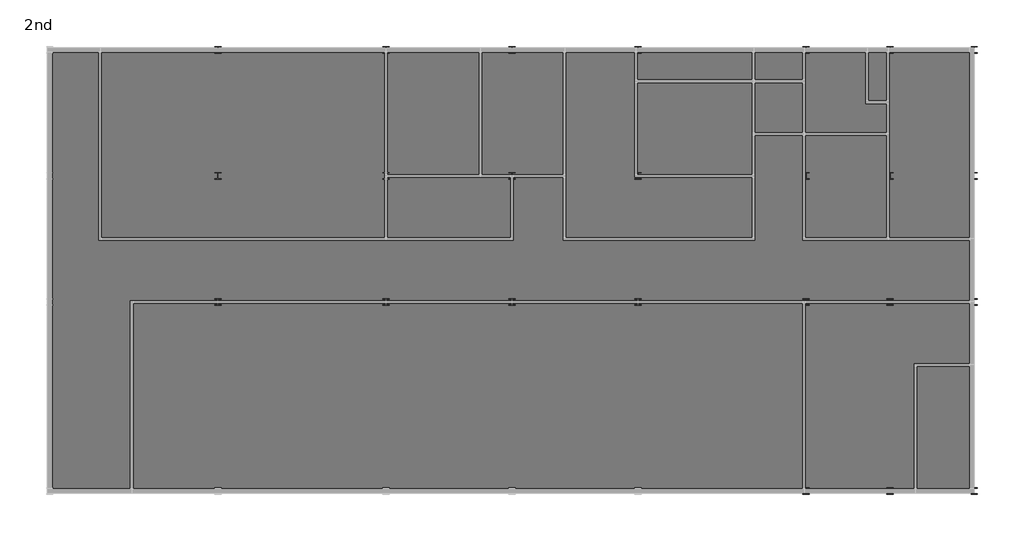
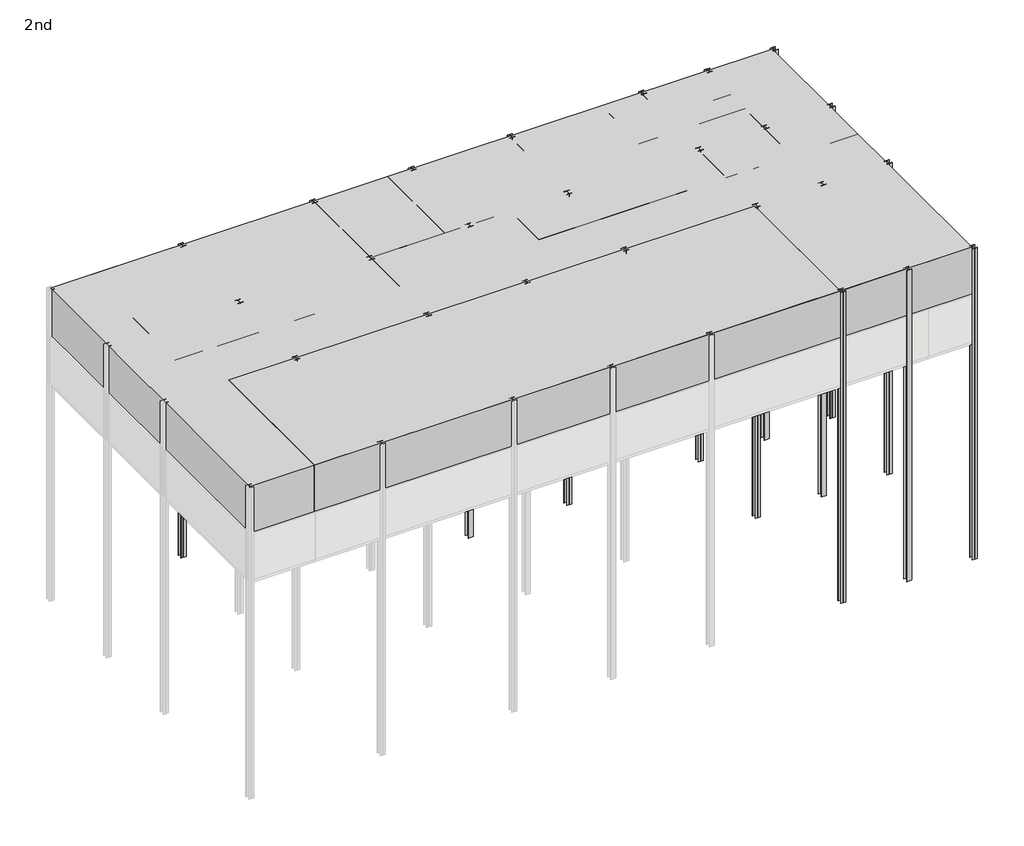
# One storey, part 3 of 3: 18 columns, 17 proxies.
"""IFC4 building model written with IfcOpenShell, lengths in millimetres."""

import ifcopenshell
import ifcopenshell.guid

model = None  # the IFC model being written
_history = None  # IfcOwnerHistory: only IFC2X3 demands one
_inside = {}  # id of a spatial element -> (the spatial element, [elements in it])
_under = {}  # id of a project, library or spatial element -> (it, [spatial elements below it])
_declared = {}  # id of a project -> (the project, [libraries it declares])
_typed = {}  # id of a type object -> (the type object, [elements of that type])
_made_of = {}  # id of a material, layer set ... -> (it, [elements and type objects made of it])


def new_model(schema):
    """Start an empty IFC model of exactly this schema.

    Asked for "IFC4X3", IfcOpenShell would pick the latest addendum, in which some entities
    have other attributes; the version numbers below select the first issue.
    IFC2X3 requires an IfcOwnerHistory on every rooted entity: one is made here for all.
    """
    global model, _history
    if schema == "IFC4X3":
        model = ifcopenshell.file(schema_version=(4, 3, 0, 0))
    else:
        model = ifcopenshell.file(schema=schema)
    _inside.clear()
    _under.clear()
    _declared.clear()
    _typed.clear()
    _made_of.clear()
    _history = None
    if model.schema == "IFC2X3":
        org = make("IfcOrganization", Name="unknown")
        user = make(
            "IfcPersonAndOrganization",
            ThePerson=make("IfcPerson", FamilyName="unknown"),
            TheOrganization=org,
        )
        app = make(
            "IfcApplication",
            ApplicationDeveloper=org,
            Version="unknown",
            ApplicationFullName="unknown",
            ApplicationIdentifier="unknown",
        )
        _history = make(
            "IfcOwnerHistory",
            OwningUser=user,
            OwningApplication=app,
            ChangeAction="ADDED",
            CreationDate=0,
        )
    return model


def make(cls, **values):
    """One entity of the class cls with the attributes given. An attribute that is None is left unset."""
    return model.create_entity(
        cls, **{name: value for name, value in values.items() if value is not None}
    )


def rooted(cls, **values):
    """An entity with a GlobalId (a new one), such as an element, a storey or a relation."""
    return make(cls, GlobalId=ifcopenshell.guid.new(), OwnerHistory=_history, **values)


def si_unit(unit_type, name, prefix=None):
    """IfcSIUnit, for example si_unit("LENGTHUNIT", "METRE", prefix="MILLI")."""
    return make("IfcSIUnit", UnitType=unit_type, Prefix=prefix, Name=name)


def assignment(units):
    """IfcUnitAssignment: the units of a project."""
    return None if units is None else make("IfcUnitAssignment", Units=units)


def point(xyz):
    """IfcCartesianPoint."""
    return None if xyz is None else make("IfcCartesianPoint", Coordinates=xyz)


def direction(xyz):
    """IfcDirection."""
    return None if xyz is None else make("IfcDirection", DirectionRatios=xyz)


def frame(location, z_axis=None, x_axis=None):
    """IfcAxis2Placement3D, a coordinate frame: its origin and axes. An axis left out is left unset."""
    return make(
        "IfcAxis2Placement3D",
        Location=point(location),
        Axis=direction(z_axis),
        RefDirection=direction(x_axis),
    )


def frame_2d(location, x_axis=None):
    """IfcAxis2Placement2D, a coordinate frame in the plane: its origin and x axis."""
    return make(
        "IfcAxis2Placement2D", Location=point(location), RefDirection=direction(x_axis)
    )


def origin():
    """The frame at (0, 0, 0) with its axes left unset."""
    return frame((0.0, 0.0, 0.0))


def origin_with_axes():
    """The frame at (0, 0, 0) with the z axis (0, 0, 1) and the x axis (1, 0, 0) written out."""
    return frame((0.0, 0.0, 0.0), z_axis=(0.0, 0.0, 1.0), x_axis=(1.0, 0.0, 0.0))


def place(relative_to, where):
    """IfcLocalPlacement: puts the frame where relative to a parent placement (None: the world)."""
    return make(
        "IfcLocalPlacement", PlacementRelTo=relative_to, RelativePlacement=where
    )


def context(
    kind, dimensions, precision=None, world=None, true_north=None, identifier=None
):
    """IfcGeometricRepresentationContext, for example the 3D "Model" context."""
    return make(
        "IfcGeometricRepresentationContext",
        ContextIdentifier=identifier,
        ContextType=kind,
        CoordinateSpaceDimension=dimensions,
        Precision=precision,
        WorldCoordinateSystem=world,
        TrueNorth=true_north,
    )


def project(units=None, contexts=None):
    """IfcProject with its units and contexts."""
    return rooted(
        "IfcProject",
        Name="project",
        RepresentationContexts=contexts,
        UnitsInContext=assignment(units),
    )


def spatial(cls, under=None, at=None, **own):
    """A site, building, storey or space (cls), placed at a placement, below another one or the project."""
    s = rooted(cls, ObjectPlacement=at, **own)
    if under is not None:
        _under.setdefault(under.id(), (under, []))[1].append(s)
    return s


def polyline(points):
    """IfcPolyline through the points."""
    return make("IfcPolyline", Points=[point(p) for p in points])


def circle_curve(where, radius):
    """IfcCircle in the frame where."""
    return make("IfcCircle", Position=where, Radius=radius)


def trimmed(basis, trim1, trim2, sense, master):
    """IfcTrimmedCurve: the piece of a basis curve between two trims."""
    return make(
        "IfcTrimmedCurve",
        BasisCurve=basis,
        Trim1=trim1,
        Trim2=trim2,
        SenseAgreement=sense,
        MasterRepresentation=master,
    )


def segment(curve, same_sense, transition):
    """IfcCompositeCurveSegment."""
    return make(
        "IfcCompositeCurveSegment",
        Transition=transition,
        SameSense=same_sense,
        ParentCurve=curve,
    )


def composite_curve(segments, self_intersect=None):
    """IfcCompositeCurve: segments joined end to end."""
    return make("IfcCompositeCurve", Segments=segments, SelfIntersect=self_intersect)


def outline(outer, holes=None, kind="AREA"):
    """IfcArbitraryClosedProfileDef: a profile drawn as a closed curve; with holes, ...WithVoids."""
    if holes is None:
        return make("IfcArbitraryClosedProfileDef", ProfileType=kind, OuterCurve=outer)
    return make(
        "IfcArbitraryProfileDefWithVoids",
        ProfileType=kind,
        OuterCurve=outer,
        InnerCurves=holes,
    )


def extrude(swept, where, along, depth):
    """IfcExtrudedAreaSolid: the profile swept, set in the frame where, extruded along a direction by depth."""
    return make(
        "IfcExtrudedAreaSolid",
        SweptArea=swept,
        Position=where,
        ExtrudedDirection=direction(along),
        Depth=depth,
    )


def shape(context_of_items, identifier, shape_type, items):
    """IfcShapeRepresentation: the items that make up one representation, for example the "Body"."""
    return make(
        "IfcShapeRepresentation",
        ContextOfItems=context_of_items,
        RepresentationIdentifier=identifier,
        RepresentationType=shape_type,
        Items=items,
    )


def source(mapping_origin, context_of_items, identifier, shape_type, items):
    """IfcRepresentationMap: a shape defined once, which mapped items show again and again."""
    return make(
        "IfcRepresentationMap",
        MappingOrigin=mapping_origin,
        MappedRepresentation=shape(context_of_items, identifier, shape_type, items),
    )


def transform(
    local_origin,
    x_axis=None,
    y_axis=None,
    z_axis=None,
    scale=None,
    scale2=None,
    scale3=None,
    uniform=True,
):
    """IfcCartesianTransformationOperator3D, or its non-uniform kind. x_axis, y_axis, z_axis: its Axis1, 2, 3."""
    if uniform:
        return make(
            "IfcCartesianTransformationOperator3D",
            Axis1=direction(x_axis),
            Axis2=direction(y_axis),
            LocalOrigin=point(local_origin),
            Scale=scale,
            Axis3=direction(z_axis),
        )
    return make(
        "IfcCartesianTransformationOperator3DnonUniform",
        Axis1=direction(x_axis),
        Axis2=direction(y_axis),
        LocalOrigin=point(local_origin),
        Scale=scale,
        Axis3=direction(z_axis),
        Scale2=scale2,
        Scale3=scale3,
    )


def mapped(mapping_source, mapping_target):
    """IfcMappedItem: shows the shape of a source again, moved by a transform."""
    return make(
        "IfcMappedItem", MappingSource=mapping_source, MappingTarget=mapping_target
    )


def made_of(thing, what):
    """Note that an element or type object is made of a material, layer set ...; save() writes the relation."""
    if what is not None:
        _made_of.setdefault(what.id(), (what, []))[1].append(thing)
    return thing


def element(
    cls,
    number,
    at=None,
    inside=None,
    cuts=None,
    type_object=None,
    material=None,
    context=None,
    identifier="Body",
    shape_type=None,
    held_by="IfcProductDefinitionShape",
    body=None,
    shapes=None,
    **own,
):
    """One element of the class cls, such as IfcWall. Its Tag is "e" and its number.

    at: its placement. inside: the storey or other place that contains it. cuts: it is an
    opening in that element (IfcRelVoidsElement). A single representation is given by context,
    identifier, shape_type and body (its items); several are given by shapes. held_by: the class
    of the entity that holds the representations. save() writes the other relations.
    """
    e = rooted(cls, Tag="e%d" % number, ObjectPlacement=at, **own)
    if body is not None:
        shapes = [shape(context, identifier, shape_type, body)]
    if shapes is not None:
        e.Representation = make(held_by, Representations=shapes)
    if inside is not None:
        _inside.setdefault(inside.id(), (inside, []))[1].append(e)
    if cuts is not None:
        rooted(
            "IfcRelVoidsElement", RelatingBuildingElement=cuts, RelatedOpeningElement=e
        )
    if type_object is not None:
        _typed.setdefault(type_object.id(), (type_object, []))[1].append(e)
    return made_of(e, material)


def aggregate(whole, parts):
    """IfcRelAggregates: a whole, such as a stair, and the parts it consists of."""
    return rooted("IfcRelAggregates", RelatingObject=whole, RelatedObjects=parts)


def save(model, path):
    """Write the relations noted so far, then the file.

    IfcRelAggregates (storeys below a building ...), IfcRelContainedInSpatialStructure (elements
    in a storey), IfcRelDefinesByType, IfcRelAssociatesMaterial and IfcRelDeclares: one each for
    every whole, place, type object, material and project.
    """
    for whole, parts in _under.values():
        aggregate(whole, parts)
    for where, things in _inside.values():
        rooted(
            "IfcRelContainedInSpatialStructure",
            RelatedElements=things,
            RelatingStructure=where,
        )
    for kind, things in _typed.values():
        rooted("IfcRelDefinesByType", RelatedObjects=things, RelatingType=kind)
    for what, things in _made_of.values():
        rooted("IfcRelAssociatesMaterial", RelatedObjects=things, RelatingMaterial=what)
    for by, libraries in _declared.values():
        rooted("IfcRelDeclares", RelatingContext=by, RelatedDefinitions=libraries)
    model.write(path)


def generic_models_29bcd6f9(model_context):
    return source(origin(), model_context, "Body", "SweptSolid", [
        extrude(outline(polyline([(2000.0, 4500.0), (2000.0, -4500.0), (-2000.0, -4500.0), (-2000.0, 4500.0), (2000.0, 4500.0)])), origin_with_axes(), (0.0, 0.0, 1.0), 6000.0),
    ])


def generic_models_5634f436(model_context):
    return source(origin(), model_context, "Body", "SweptSolid", [
        extrude(outline(polyline([(1350.0, 3000.0), (1350.0, -3000.0), (-1350.0, -3000.0), (-1350.0, 3000.0), (1350.0, 3000.0)])), origin_with_axes(), (0.0, 0.0, 1.0), 6000.0),
    ])


def generic_models_71e2440f(model_context):
    return source(origin(), model_context, "Body", "SweptSolid", [
        extrude(outline(polyline([(500.0, 1250.0), (500.0, -1250.0), (-500.0, -1250.0), (-500.0, 1250.0), (500.0, 1250.0)])), origin_with_axes(), (0.0, 0.0, 1.0), 6000.0),
    ])


def generic_models_57c7875f(model_context):
    return source(origin(), model_context, "Body", "SweptSolid", [
        extrude(outline(polyline([(4500.0, 16000.0), (4500.0, -16000.0), (-4500.0, -16000.0), (-4500.0, 16000.0), (4500.0, 16000.0)])), origin_with_axes(), (0.0, 0.0, 1.0), 6000.0),
    ])


def generic_models_7bff30ad(model_context):
    return source(origin(), model_context, "Body", "SweptSolid", [
        extrude(outline(polyline([(2000.0, 2000.0), (2000.0, -2000.0), (-2000.0, -2000.0), (-2000.0, 2000.0), (2000.0, 2000.0)])), origin_with_axes(), (0.0, 0.0, 1.0), 6000.0),
    ])


def generic_models_5b7b272c(model_context):
    return source(origin(), model_context, "Body", "SweptSolid", [
        extrude(outline(polyline([(2000.0, 2500.0), (2000.0, -2500.0), (-2000.0, -2500.0), (-2000.0, 2500.0), (2000.0, 2500.0)])), origin_with_axes(), (0.0, 0.0, 1.0), 6000.0),
    ])


def generic_models_47b98be1(model_context):
    return source(origin(), model_context, "Body", "SweptSolid", [
        extrude(outline(polyline([(1200.0, 2000.0), (1200.0, -2000.0), (-1200.0, -2000.0), (-1200.0, 2000.0), (1200.0, 2000.0)])), origin_with_axes(), (0.0, 0.0, 1.0), 6000.0),
    ])


def generic_models_7a053eeb(model_context):
    return source(origin(), model_context, "Body", "SweptSolid", [
        extrude(outline(polyline([(1200.0, 750.0), (1200.0, -750.0), (-1200.0, -750.0), (-1200.0, 750.0), (1200.0, 750.0)])), origin_with_axes(), (0.0, 0.0, 1.0), 6000.0),
    ])


def generic_models_ec17d728(model_context):
    return source(origin(), model_context, "Body", "SweptSolid", [
        extrude(outline(polyline([(2800.0, 3000.0), (2800.0, -3000.0), (-2800.0, -3000.0), (-2800.0, 3000.0), (2800.0, 3000.0)])), origin_with_axes(), (0.0, 0.0, 1.0), 6000.0),
    ])


def generic_models_85897e09(model_context):
    return source(origin(), model_context, "Body", "SweptSolid", [
        extrude(outline(polyline([(2800.0, 750.0), (2800.0, -750.0), (-2800.0, -750.0), (-2800.0, 750.0), (2800.0, 750.0)])), origin_with_axes(), (0.0, 0.0, 1.0), 6000.0),
    ])


def generic_models_b79df083(model_context):
    return source(origin(), model_context, "Body", "SweptSolid", [
        extrude(outline(polyline([(4500.0, 4500.0), (4500.0, -4500.0), (-4500.0, -4500.0), (-4500.0, 4500.0), (4500.0, 4500.0)])), origin_with_axes(), (0.0, 0.0, 1.0), 6000.0),
    ])


def generic_models_98b71764(model_context):
    return source(origin(), model_context, "Body", "SweptSolid", [
        extrude(outline(polyline([(2000.0, 3000.0), (2000.0, -3000.0), (-2000.0, -3000.0), (-2000.0, 3000.0), (2000.0, 3000.0)])), origin_with_axes(), (0.0, 0.0, 1.0), 6000.0),
    ])


def generic_models_8af91fed(model_context):
    return source(origin(), model_context, "Body", "SweptSolid", [
        extrude(outline(polyline([(2250.0, 3000.0), (2250.0, -3000.0), (-2250.0, -3000.0), (-2250.0, 3000.0), (2250.0, 3000.0)])), origin_with_axes(), (0.0, 0.0, 1.0), 6000.0),
    ])


def generic_models_542cc789(model_context):
    return source(origin(), model_context, "Body", "SweptSolid", [
        extrude(outline(polyline([(1500.0, 3000.0), (1500.0, -3000.0), (-1500.0, -3000.0), (-1500.0, 3000.0), (1500.0, 3000.0)])), origin_with_axes(), (0.0, 0.0, 1.0), 6000.0),
    ])


def generic_models_af0009da(model_context):
    return source(origin(), model_context, "Body", "SweptSolid", [
        extrude(outline(polyline([(4500.0, 6800.0), (4500.0, -6800.0), (-4500.0, -6800.0), (-4500.0, 6800.0), (4500.0, 6800.0)])), origin_with_axes(), (0.0, 0.0, 1.0), 6000.0),
    ])


def generic_models_4d084078(model_context):
    return source(origin(), model_context, "Body", "SweptSolid", [
        extrude(outline(polyline([(4000.0, 4500.0), (4000.0, -4500.0), (-4000.0, -4500.0), (-4000.0, 4500.0), (4000.0, 4500.0)])), origin_with_axes(), (0.0, 0.0, 1.0), 6000.0),
    ])


def generic_models_b3b0fa1d(model_context):
    return source(origin(), model_context, "Body", "SweptSolid", [
        extrude(outline(polyline([(21950.0, 10500.0), (21950.0, -10500.0), (-21950.0, -10500.0), (-21950.0, 10500.0), (21950.0, 10500.0)])), origin_with_axes(), (0.0, 0.0, 1.0), 6000.0),
    ])


model = new_model("IFC4")

# Units and contexts
model_context = context("Model", 3, world=origin())
ifc_project = project(units=[si_unit("LENGTHUNIT", "METRE", prefix="MILLI")], contexts=[model_context])

# Site, building, storey
site = spatial("IfcSite", under=ifc_project)
building = spatial("IfcBuilding", under=site)
storey = spatial("IfcBuildingStorey", under=building, Name="2nd", Elevation=14000.0)

# Proxies
placement = place(None, origin())
generic_models_shape = generic_models_29bcd6f9(model_context)
element("IfcBuildingElementProxy", 1, Name="Space Planning Box_hec : Space Planning Box_hec", ObjectType="Space Planning Box_hec : Space Planning Box_hec", at=placement, inside=storey, context=model_context, shape_type="MappedRepresentation", body=[
    mapped(generic_models_shape, transform((198014.1020501, 147515.7581198, 14000.0), x_axis=(1.0, 0.0, 0.0), y_axis=(0.0, 1.0, 0.0), z_axis=(0.0, 0.0, 1.0))),
])
generic_models_2_shape = generic_models_5634f436(model_context)
element("IfcBuildingElementProxy", 2, Name="Space Planning Box_hec : Space Planning Box_hec", ObjectType="Space Planning Box_hec : Space Planning Box_hec", at=placement, inside=storey, context=model_context, shape_type="MappedRepresentation", body=[
    mapped(generic_models_2_shape, transform((198664.1020501, 134015.7581198, 14000.0), x_axis=(1.0, 0.0, 0.0), y_axis=(0.0, 1.0, 0.0), z_axis=(0.0, 0.0, 1.0))),
])
generic_models_3_shape = generic_models_71e2440f(model_context)
element("IfcBuildingElementProxy", 3, Name="Space Planning Box_hec : Space Planning Box_hec", ObjectType="Space Planning Box_hec : Space Planning Box_hec", at=placement, inside=storey, context=model_context, shape_type="MappedRepresentation", body=[
    mapped(generic_models_3_shape, transform((195514.1020501, 150765.7581198, 14000.0), x_axis=(1.0, 0.0, 0.0), y_axis=(0.0, 1.0, 0.0), z_axis=(0.0, 0.0, 1.0))),
])
generic_models_4_shape = generic_models_57c7875f(model_context)
element("IfcBuildingElementProxy", 4, Name="Space Planning Box_hec : Space Planning Box_hec", ObjectType="Space Planning Box_hec : Space Planning Box_hec", at=placement, inside=storey, context=model_context, shape_type="MappedRepresentation", body=[
    mapped(generic_models_4_shape, transform((176014.1020501, 135515.7581198, 14000.0), x_axis=(0.0, -1.0, 0.0), y_axis=(1.0, 0.0, 0.0), z_axis=(0.0, 0.0, 1.0))),
])
generic_models_5_shape = generic_models_7bff30ad(model_context)
element("IfcBuildingElementProxy", 5, Name="Space Planning Box_hec : Space Planning Box_hec", ObjectType="Space Planning Box_hec : Space Planning Box_hec", at=placement, inside=storey, context=model_context, shape_type="MappedRepresentation", body=[
    mapped(generic_models_5_shape, transform((194014.1020501, 150015.7581198, 14000.0), x_axis=(1.0, 0.0, 0.0), y_axis=(0.0, 1.0, 0.0), z_axis=(0.0, 0.0, 1.0))),
])
generic_models_6_shape = generic_models_5b7b272c(model_context)
element("IfcBuildingElementProxy", 6, Name="Space Planning Box_hec : Space Planning Box_hec", ObjectType="Space Planning Box_hec : Space Planning Box_hec", at=placement, inside=storey, context=model_context, shape_type="MappedRepresentation", body=[
    mapped(generic_models_6_shape, transform((194014.1020501, 145515.7581198, 14000.0), x_axis=(1.0, 0.0, 0.0), y_axis=(0.0, 1.0, 0.0), z_axis=(0.0, 0.0, 1.0))),
])
generic_models_7_shape = generic_models_47b98be1(model_context)
element("IfcBuildingElementProxy", 7, Name="Space Planning Box_hec : Space Planning Box_hec", ObjectType="Space Planning Box_hec : Space Planning Box_hec", at=placement, inside=storey, context=model_context, shape_type="MappedRepresentation", body=[
    mapped(generic_models_7_shape, transform((190814.1020501, 150015.7581198, 14000.0), x_axis=(1.0, 0.0, 0.0), y_axis=(0.0, 1.0, 0.0), z_axis=(0.0, 0.0, 1.0))),
])
generic_models_8_shape = generic_models_7a053eeb(model_context)
element("IfcBuildingElementProxy", 8, Name="Space Planning Box_hec : Space Planning Box_hec", ObjectType="Space Planning Box_hec : Space Planning Box_hec", at=placement, inside=storey, context=model_context, shape_type="MappedRepresentation", body=[
    mapped(generic_models_8_shape, transform((190814.1020501, 151265.7581198, 14000.0), x_axis=(1.0, 0.0, 0.0), y_axis=(0.0, 1.0, 0.0), z_axis=(0.0, 0.0, 1.0))),
])
generic_models_9_shape = generic_models_ec17d728(model_context)
element("IfcBuildingElementProxy", 9, Name="Space Planning Box_hec : Space Planning Box_hec", ObjectType="Space Planning Box_hec : Space Planning Box_hec", at=placement, inside=storey, context=model_context, shape_type="MappedRepresentation", body=[
    mapped(generic_models_9_shape, transform((186814.1020501, 149015.7581198, 14000.0), x_axis=(1.0, 0.0, 0.0), y_axis=(0.0, 1.0, 0.0), z_axis=(0.0, 0.0, 1.0))),
])
generic_models_10_shape = generic_models_85897e09(model_context)
element("IfcBuildingElementProxy", 10, Name="Space Planning Box_hec : Space Planning Box_hec", ObjectType="Space Planning Box_hec : Space Planning Box_hec", at=placement, inside=storey, context=model_context, shape_type="MappedRepresentation", body=[
    mapped(generic_models_10_shape, transform((186814.1020501, 151265.7581198, 14000.0), x_axis=(1.0, 0.0, 0.0), y_axis=(0.0, 1.0, 0.0), z_axis=(0.0, 0.0, 1.0))),
])
generic_models_11_shape = generic_models_b79df083(model_context)
element("IfcBuildingElementProxy", 11, Name="Space Planning Box_hec : Space Planning Box_hec", ObjectType="Space Planning Box_hec : Space Planning Box_hec", at=placement, inside=storey, context=model_context, shape_type="MappedRepresentation", body=[
    mapped(generic_models_11_shape, transform((185114.1020501, 147515.7581198, 14000.0), x_axis=(1.0, 0.0, 0.0), y_axis=(0.0, 1.0, 0.0), z_axis=(0.0, 0.0, 1.0))),
])
generic_models_12_shape = generic_models_98b71764(model_context)
element("IfcBuildingElementProxy", 12, Name="Space Planning Box_hec : Space Planning Box_hec", ObjectType="Space Planning Box_hec : Space Planning Box_hec", at=placement, inside=storey, context=model_context, shape_type="MappedRepresentation", body=[
    mapped(generic_models_12_shape, transform((178614.1020501, 149015.7581198, 14000.0), x_axis=(1.0, 0.0, 0.0), y_axis=(0.0, 1.0, 0.0), z_axis=(0.0, 0.0, 1.0))),
])
generic_models_13_shape = generic_models_8af91fed(model_context)
element("IfcBuildingElementProxy", 13, Name="Space Planning Box_hec : Space Planning Box_hec", ObjectType="Space Planning Box_hec : Space Planning Box_hec", at=placement, inside=storey, context=model_context, shape_type="MappedRepresentation", body=[
    mapped(generic_models_13_shape, transform((174364.1020501, 149015.7581198, 14000.0), x_axis=(1.0, 0.0, 0.0), y_axis=(0.0, 1.0, 0.0), z_axis=(0.0, 0.0, 1.0))),
])
generic_models_14_shape = generic_models_542cc789(model_context)
element("IfcBuildingElementProxy", 14, Name="Space Planning Box_hec : Space Planning Box_hec", ObjectType="Space Planning Box_hec : Space Planning Box_hec", at=placement, inside=storey, context=model_context, shape_type="MappedRepresentation", body=[
    mapped(generic_models_14_shape, transform((175114.1020501, 144515.7581198, 14000.0), x_axis=(0.0, 1.0, 0.0), y_axis=(-1.0, 0.0, 0.0), z_axis=(0.0, 0.0, 1.0))),
])
generic_models_15_shape = generic_models_af0009da(model_context)
element("IfcBuildingElementProxy", 15, Name="Space Planning Box_hec : Space Planning Box_hec", ObjectType="Space Planning Box_hec : Space Planning Box_hec", at=placement, inside=storey, context=model_context, shape_type="MappedRepresentation", body=[
    mapped(generic_models_15_shape, transform((165314.1020501, 147515.7581198, 14000.0), x_axis=(0.0, -1.0, 0.0), y_axis=(1.0, 0.0, 0.0), z_axis=(0.0, 0.0, 1.0))),
])
generic_models_16_shape = generic_models_4d084078(model_context)
element("IfcBuildingElementProxy", 16, Name="Space Planning Box_hec : Space Planning Box_hec", ObjectType="Space Planning Box_hec : Space Planning Box_hec", at=placement, inside=storey, context=model_context, shape_type="MappedRepresentation", body=[
    mapped(generic_models_16_shape, transform((196014.1020501, 135515.7581198, 14000.0), x_axis=(1.0, 0.0, 0.0), y_axis=(0.0, 1.0, 0.0), z_axis=(0.0, 0.0, 1.0))),
])
generic_models_17_shape = generic_models_b3b0fa1d(model_context)
element("IfcBuildingElementProxy", 17, Name="Space Planning Box_hec : Space Planning Box_hec", ObjectType="Space Planning Box_hec : Space Planning Box_hec", at=placement, inside=storey, context=model_context, shape_type="MappedRepresentation", body=[
    mapped(generic_models_17_shape, transform((178064.1020501, 141515.7581198, 14000.0), x_axis=(1.0, 0.0, 0.0), y_axis=(0.0, 1.0, 0.0), z_axis=(0.0, 0.0, 1.0))),
])

# Columns
element("IfcColumn", 18, ObjectType="UC-Universal Columns-Column : UC305x305x97", at=placement, inside=storey, context=model_context, shape_type="SweptSolid", body=[
    extrude(outline(composite_curve([segment(polyline([(164266.7520501, 152169.7081198), (164266.7520501, 152154.3081198), (164134.2520501, 152154.3081198)]), True, "CONTINUOUS"), segment(trimmed(circle_curve(frame_2d((164134.2520501, 152139.1081198)), 15.2), [point((164134.2520501, 152154.3081198))], [point((164119.0520501, 152139.1081198))], True, "CARTESIAN"), True, "CONTINUOUS"), segment(polyline([(164119.0520501, 152139.1081198), (164119.0520501, 151892.4081198)]), True, "CONTINUOUS"), segment(trimmed(circle_curve(frame_2d((164134.2520501, 151892.4081198)), 15.2), [point((164119.0520501, 151892.4081198))], [point((164134.2520501, 151877.2081198))], True, "CARTESIAN"), True, "CONTINUOUS"), segment(polyline([(164134.2520501, 151877.2081198), (164266.7520501, 151877.2081198), (164266.7520501, 151861.8081198), (163961.4520501, 151861.8081198), (163961.4520501, 151877.2081198), (164093.9520501, 151877.2081198)]), True, "CONTINUOUS"), segment(trimmed(circle_curve(frame_2d((164093.9520501, 151892.4081198)), 15.2), [point((164093.9520501, 151877.2081198))], [point((164109.1520501, 151892.4081198))], True, "CARTESIAN"), True, "CONTINUOUS"), segment(polyline([(164109.1520501, 151892.4081198), (164109.1520501, 152139.1081198)]), True, "CONTINUOUS"), segment(trimmed(circle_curve(frame_2d((164093.9520501, 152139.1081198)), 15.2), [point((164109.1520501, 152139.1081198))], [point((164093.9520501, 152154.3081198))], True, "CARTESIAN"), True, "CONTINUOUS"), segment(polyline([(164093.9520501, 152154.3081198), (163961.4520501, 152154.3081198), (163961.4520501, 152169.7081198), (164266.7520501, 152169.7081198)]), True, "CONTINUOUS")], self_intersect=False)), origin_with_axes(), (0.0, 0.0, 1.0), 20000.0),
])
element("IfcColumn", 19, ObjectType="UC-Universal Columns-Column : UC305x305x97", at=placement, inside=storey, context=model_context, shape_type="SweptSolid", body=[
    extrude(outline(composite_curve([segment(polyline([(172266.7520501, 152169.7081198), (172266.7520501, 152154.3081198), (172134.2520501, 152154.3081198)]), True, "CONTINUOUS"), segment(trimmed(circle_curve(frame_2d((172134.2520501, 152139.1081198)), 15.2), [point((172134.2520501, 152154.3081198))], [point((172119.0520501, 152139.1081198))], True, "CARTESIAN"), True, "CONTINUOUS"), segment(polyline([(172119.0520501, 152139.1081198), (172119.0520501, 151892.4081198)]), True, "CONTINUOUS"), segment(trimmed(circle_curve(frame_2d((172134.2520501, 151892.4081198)), 15.2), [point((172119.0520501, 151892.4081198))], [point((172134.2520501, 151877.2081198))], True, "CARTESIAN"), True, "CONTINUOUS"), segment(polyline([(172134.2520501, 151877.2081198), (172266.7520501, 151877.2081198), (172266.7520501, 151861.8081198), (171961.4520501, 151861.8081198), (171961.4520501, 151877.2081198), (172093.9520501, 151877.2081198)]), True, "CONTINUOUS"), segment(trimmed(circle_curve(frame_2d((172093.9520501, 151892.4081198)), 15.2), [point((172093.9520501, 151877.2081198))], [point((172109.1520501, 151892.4081198))], True, "CARTESIAN"), True, "CONTINUOUS"), segment(polyline([(172109.1520501, 151892.4081198), (172109.1520501, 152139.1081198)]), True, "CONTINUOUS"), segment(trimmed(circle_curve(frame_2d((172093.9520501, 152139.1081198)), 15.2), [point((172109.1520501, 152139.1081198))], [point((172093.9520501, 152154.3081198))], True, "CARTESIAN"), True, "CONTINUOUS"), segment(polyline([(172093.9520501, 152154.3081198), (171961.4520501, 152154.3081198), (171961.4520501, 152169.7081198), (172266.7520501, 152169.7081198)]), True, "CONTINUOUS")], self_intersect=False)), origin_with_axes(), (0.0, 0.0, 1.0), 20000.0),
])
element("IfcColumn", 20, ObjectType="UC-Universal Columns-Column : UC305x305x97", at=placement, inside=storey, context=model_context, shape_type="SweptSolid", body=[
    extrude(outline(composite_curve([segment(polyline([(178266.7520501, 152169.7081198), (178266.7520501, 152154.3081198), (178134.2520501, 152154.3081198)]), True, "CONTINUOUS"), segment(trimmed(circle_curve(frame_2d((178134.2520501, 152139.1081198)), 15.2), [point((178134.2520501, 152154.3081198))], [point((178119.0520501, 152139.1081198))], True, "CARTESIAN"), True, "CONTINUOUS"), segment(polyline([(178119.0520501, 152139.1081198), (178119.0520501, 151892.4081198)]), True, "CONTINUOUS"), segment(trimmed(circle_curve(frame_2d((178134.2520501, 151892.4081198)), 15.2), [point((178119.0520501, 151892.4081198))], [point((178134.2520501, 151877.2081198))], True, "CARTESIAN"), True, "CONTINUOUS"), segment(polyline([(178134.2520501, 151877.2081198), (178266.7520501, 151877.2081198), (178266.7520501, 151861.8081198), (177961.4520501, 151861.8081198), (177961.4520501, 151877.2081198), (178093.9520501, 151877.2081198)]), True, "CONTINUOUS"), segment(trimmed(circle_curve(frame_2d((178093.9520501, 151892.4081198)), 15.2), [point((178093.9520501, 151877.2081198))], [point((178109.1520501, 151892.4081198))], True, "CARTESIAN"), True, "CONTINUOUS"), segment(polyline([(178109.1520501, 151892.4081198), (178109.1520501, 152139.1081198)]), True, "CONTINUOUS"), segment(trimmed(circle_curve(frame_2d((178093.9520501, 152139.1081198)), 15.2), [point((178109.1520501, 152139.1081198))], [point((178093.9520501, 152154.3081198))], True, "CARTESIAN"), True, "CONTINUOUS"), segment(polyline([(178093.9520501, 152154.3081198), (177961.4520501, 152154.3081198), (177961.4520501, 152169.7081198), (178266.7520501, 152169.7081198)]), True, "CONTINUOUS")], self_intersect=False)), origin_with_axes(), (0.0, 0.0, 1.0), 20000.0),
])
element("IfcColumn", 21, ObjectType="UC-Universal Columns-Column : UC305x305x97", at=placement, inside=storey, context=model_context, shape_type="SweptSolid", body=[
    extrude(outline(composite_curve([segment(polyline([(178266.7520501, 146169.7081198), (178266.7520501, 146154.3081198), (178134.2520501, 146154.3081198)]), True, "CONTINUOUS"), segment(trimmed(circle_curve(frame_2d((178134.2520501, 146139.1081198)), 15.2), [point((178134.2520501, 146154.3081198))], [point((178119.0520501, 146139.1081198))], True, "CARTESIAN"), True, "CONTINUOUS"), segment(polyline([(178119.0520501, 146139.1081198), (178119.0520501, 145892.4081198)]), True, "CONTINUOUS"), segment(trimmed(circle_curve(frame_2d((178134.2520501, 145892.4081198)), 15.2), [point((178119.0520501, 145892.4081198))], [point((178134.2520501, 145877.2081198))], True, "CARTESIAN"), True, "CONTINUOUS"), segment(polyline([(178134.2520501, 145877.2081198), (178266.7520501, 145877.2081198), (178266.7520501, 145861.8081198), (177961.4520501, 145861.8081198), (177961.4520501, 145877.2081198), (178093.9520501, 145877.2081198)]), True, "CONTINUOUS"), segment(trimmed(circle_curve(frame_2d((178093.9520501, 145892.4081198)), 15.2), [point((178093.9520501, 145877.2081198))], [point((178109.1520501, 145892.4081198))], True, "CARTESIAN"), True, "CONTINUOUS"), segment(polyline([(178109.1520501, 145892.4081198), (178109.1520501, 146139.1081198)]), True, "CONTINUOUS"), segment(trimmed(circle_curve(frame_2d((178093.9520501, 146139.1081198)), 15.2), [point((178109.1520501, 146139.1081198))], [point((178093.9520501, 146154.3081198))], True, "CARTESIAN"), True, "CONTINUOUS"), segment(polyline([(178093.9520501, 146154.3081198), (177961.4520501, 146154.3081198), (177961.4520501, 146169.7081198), (178266.7520501, 146169.7081198)]), True, "CONTINUOUS")], self_intersect=False)), origin_with_axes(), (0.0, 0.0, 1.0), 20000.0),
])
element("IfcColumn", 22, ObjectType="UC-Universal Columns-Column : UC305x305x97", at=placement, inside=storey, context=model_context, shape_type="SweptSolid", body=[
    extrude(outline(composite_curve([segment(polyline([(184266.7520501, 152169.7081198), (184266.7520501, 152154.3081198), (184134.2520501, 152154.3081198)]), True, "CONTINUOUS"), segment(trimmed(circle_curve(frame_2d((184134.2520501, 152139.1081198)), 15.2), [point((184134.2520501, 152154.3081198))], [point((184119.0520501, 152139.1081198))], True, "CARTESIAN"), True, "CONTINUOUS"), segment(polyline([(184119.0520501, 152139.1081198), (184119.0520501, 151892.4081198)]), True, "CONTINUOUS"), segment(trimmed(circle_curve(frame_2d((184134.2520501, 151892.4081198)), 15.2), [point((184119.0520501, 151892.4081198))], [point((184134.2520501, 151877.2081198))], True, "CARTESIAN"), True, "CONTINUOUS"), segment(polyline([(184134.2520501, 151877.2081198), (184266.7520501, 151877.2081198), (184266.7520501, 151861.8081198), (183961.4520501, 151861.8081198), (183961.4520501, 151877.2081198), (184093.9520501, 151877.2081198)]), True, "CONTINUOUS"), segment(trimmed(circle_curve(frame_2d((184093.9520501, 151892.4081198)), 15.2), [point((184093.9520501, 151877.2081198))], [point((184109.1520501, 151892.4081198))], True, "CARTESIAN"), True, "CONTINUOUS"), segment(polyline([(184109.1520501, 151892.4081198), (184109.1520501, 152139.1081198)]), True, "CONTINUOUS"), segment(trimmed(circle_curve(frame_2d((184093.9520501, 152139.1081198)), 15.2), [point((184109.1520501, 152139.1081198))], [point((184093.9520501, 152154.3081198))], True, "CARTESIAN"), True, "CONTINUOUS"), segment(polyline([(184093.9520501, 152154.3081198), (183961.4520501, 152154.3081198), (183961.4520501, 152169.7081198), (184266.7520501, 152169.7081198)]), True, "CONTINUOUS")], self_intersect=False)), origin_with_axes(), (0.0, 0.0, 1.0), 20000.0),
])
element("IfcColumn", 23, ObjectType="UC-Universal Columns-Column : UC305x305x97", at=placement, inside=storey, context=model_context, shape_type="SweptSolid", body=[
    extrude(outline(composite_curve([segment(polyline([(184266.7520501, 146169.7081198), (184266.7520501, 146154.3081198), (184134.2520501, 146154.3081198)]), True, "CONTINUOUS"), segment(trimmed(circle_curve(frame_2d((184134.2520501, 146139.1081198)), 15.2), [point((184134.2520501, 146154.3081198))], [point((184119.0520501, 146139.1081198))], True, "CARTESIAN"), True, "CONTINUOUS"), segment(polyline([(184119.0520501, 146139.1081198), (184119.0520501, 145892.4081198)]), True, "CONTINUOUS"), segment(trimmed(circle_curve(frame_2d((184134.2520501, 145892.4081198)), 15.2), [point((184119.0520501, 145892.4081198))], [point((184134.2520501, 145877.2081198))], True, "CARTESIAN"), True, "CONTINUOUS"), segment(polyline([(184134.2520501, 145877.2081198), (184266.7520501, 145877.2081198), (184266.7520501, 145861.8081198), (183961.4520501, 145861.8081198), (183961.4520501, 145877.2081198), (184093.9520501, 145877.2081198)]), True, "CONTINUOUS"), segment(trimmed(circle_curve(frame_2d((184093.9520501, 145892.4081198)), 15.2), [point((184093.9520501, 145877.2081198))], [point((184109.1520501, 145892.4081198))], True, "CARTESIAN"), True, "CONTINUOUS"), segment(polyline([(184109.1520501, 145892.4081198), (184109.1520501, 146139.1081198)]), True, "CONTINUOUS"), segment(trimmed(circle_curve(frame_2d((184093.9520501, 146139.1081198)), 15.2), [point((184109.1520501, 146139.1081198))], [point((184093.9520501, 146154.3081198))], True, "CARTESIAN"), True, "CONTINUOUS"), segment(polyline([(184093.9520501, 146154.3081198), (183961.4520501, 146154.3081198), (183961.4520501, 146169.7081198), (184266.7520501, 146169.7081198)]), True, "CONTINUOUS")], self_intersect=False)), origin_with_axes(), (0.0, 0.0, 1.0), 20000.0),
])
element("IfcColumn", 24, ObjectType="UC-Universal Columns-Column : UC305x305x97", at=placement, inside=storey, context=model_context, shape_type="SweptSolid", body=[
    extrude(outline(composite_curve([segment(polyline([(192266.7520501, 152169.7081198), (192266.7520501, 152154.3081198), (192134.2520501, 152154.3081198)]), True, "CONTINUOUS"), segment(trimmed(circle_curve(frame_2d((192134.2520501, 152139.1081198)), 15.2), [point((192134.2520501, 152154.3081198))], [point((192119.0520501, 152139.1081198))], True, "CARTESIAN"), True, "CONTINUOUS"), segment(polyline([(192119.0520501, 152139.1081198), (192119.0520501, 151892.4081198)]), True, "CONTINUOUS"), segment(trimmed(circle_curve(frame_2d((192134.2520501, 151892.4081198)), 15.2), [point((192119.0520501, 151892.4081198))], [point((192134.2520501, 151877.2081198))], True, "CARTESIAN"), True, "CONTINUOUS"), segment(polyline([(192134.2520501, 151877.2081198), (192266.7520501, 151877.2081198), (192266.7520501, 151861.8081198), (191961.4520501, 151861.8081198), (191961.4520501, 151877.2081198), (192093.9520501, 151877.2081198)]), True, "CONTINUOUS"), segment(trimmed(circle_curve(frame_2d((192093.9520501, 151892.4081198)), 15.2), [point((192093.9520501, 151877.2081198))], [point((192109.1520501, 151892.4081198))], True, "CARTESIAN"), True, "CONTINUOUS"), segment(polyline([(192109.1520501, 151892.4081198), (192109.1520501, 152139.1081198)]), True, "CONTINUOUS"), segment(trimmed(circle_curve(frame_2d((192093.9520501, 152139.1081198)), 15.2), [point((192109.1520501, 152139.1081198))], [point((192093.9520501, 152154.3081198))], True, "CARTESIAN"), True, "CONTINUOUS"), segment(polyline([(192093.9520501, 152154.3081198), (191961.4520501, 152154.3081198), (191961.4520501, 152169.7081198), (192266.7520501, 152169.7081198)]), True, "CONTINUOUS")], self_intersect=False)), origin_with_axes(), (0.0, 0.0, 1.0), 20000.0),
])
element("IfcColumn", 25, ObjectType="UC-Universal Columns-Column : UC305x305x97", at=placement, inside=storey, context=model_context, shape_type="SweptSolid", body=[
    extrude(outline(composite_curve([segment(polyline([(192266.7520501, 146169.7081198), (192266.7520501, 146154.3081198), (192134.2520501, 146154.3081198)]), True, "CONTINUOUS"), segment(trimmed(circle_curve(frame_2d((192134.2520501, 146139.1081198)), 15.2), [point((192134.2520501, 146154.3081198))], [point((192119.0520501, 146139.1081198))], True, "CARTESIAN"), True, "CONTINUOUS"), segment(polyline([(192119.0520501, 146139.1081198), (192119.0520501, 145892.4081198)]), True, "CONTINUOUS"), segment(trimmed(circle_curve(frame_2d((192134.2520501, 145892.4081198)), 15.2), [point((192119.0520501, 145892.4081198))], [point((192134.2520501, 145877.2081198))], True, "CARTESIAN"), True, "CONTINUOUS"), segment(polyline([(192134.2520501, 145877.2081198), (192266.7520501, 145877.2081198), (192266.7520501, 145861.8081198), (191961.4520501, 145861.8081198), (191961.4520501, 145877.2081198), (192093.9520501, 145877.2081198)]), True, "CONTINUOUS"), segment(trimmed(circle_curve(frame_2d((192093.9520501, 145892.4081198)), 15.2), [point((192093.9520501, 145877.2081198))], [point((192109.1520501, 145892.4081198))], True, "CARTESIAN"), True, "CONTINUOUS"), segment(polyline([(192109.1520501, 145892.4081198), (192109.1520501, 146139.1081198)]), True, "CONTINUOUS"), segment(trimmed(circle_curve(frame_2d((192093.9520501, 146139.1081198)), 15.2), [point((192109.1520501, 146139.1081198))], [point((192093.9520501, 146154.3081198))], True, "CARTESIAN"), True, "CONTINUOUS"), segment(polyline([(192093.9520501, 146154.3081198), (191961.4520501, 146154.3081198), (191961.4520501, 146169.7081198), (192266.7520501, 146169.7081198)]), True, "CONTINUOUS")], self_intersect=False)), origin_with_axes(), (0.0, 0.0, 1.0), 20000.0),
])
element("IfcColumn", 26, ObjectType="UC-Universal Columns-Column : UC305x305x97", at=placement, inside=storey, context=model_context, shape_type="SweptSolid", body=[
    extrude(outline(composite_curve([segment(polyline([(192266.7520501, 140169.7081198), (192266.7520501, 140154.3081198), (192134.2520501, 140154.3081198)]), True, "CONTINUOUS"), segment(trimmed(circle_curve(frame_2d((192134.2520501, 140139.1081198)), 15.2), [point((192134.2520501, 140154.3081198))], [point((192119.0520501, 140139.1081198))], True, "CARTESIAN"), True, "CONTINUOUS"), segment(polyline([(192119.0520501, 140139.1081198), (192119.0520501, 139892.4081198)]), True, "CONTINUOUS"), segment(trimmed(circle_curve(frame_2d((192134.2520501, 139892.4081198)), 15.2), [point((192119.0520501, 139892.4081198))], [point((192134.2520501, 139877.2081198))], True, "CARTESIAN"), True, "CONTINUOUS"), segment(polyline([(192134.2520501, 139877.2081198), (192266.7520501, 139877.2081198), (192266.7520501, 139861.8081198), (191961.4520501, 139861.8081198), (191961.4520501, 139877.2081198), (192093.9520501, 139877.2081198)]), True, "CONTINUOUS"), segment(trimmed(circle_curve(frame_2d((192093.9520501, 139892.4081198)), 15.2), [point((192093.9520501, 139877.2081198))], [point((192109.1520501, 139892.4081198))], True, "CARTESIAN"), True, "CONTINUOUS"), segment(polyline([(192109.1520501, 139892.4081198), (192109.1520501, 140139.1081198)]), True, "CONTINUOUS"), segment(trimmed(circle_curve(frame_2d((192093.9520501, 140139.1081198)), 15.2), [point((192109.1520501, 140139.1081198))], [point((192093.9520501, 140154.3081198))], True, "CARTESIAN"), True, "CONTINUOUS"), segment(polyline([(192093.9520501, 140154.3081198), (191961.4520501, 140154.3081198), (191961.4520501, 140169.7081198), (192266.7520501, 140169.7081198)]), True, "CONTINUOUS")], self_intersect=False)), origin_with_axes(), (0.0, 0.0, 1.0), 20000.0),
])
element("IfcColumn", 27, ObjectType="UC-Universal Columns-Column : UC305x305x97", at=placement, inside=storey, context=model_context, shape_type="SweptSolid", body=[
    extrude(outline(composite_curve([segment(polyline([(192266.7520501, 131169.7081198), (192266.7520501, 131154.3081198), (192134.2520501, 131154.3081198)]), True, "CONTINUOUS"), segment(trimmed(circle_curve(frame_2d((192134.2520501, 131139.1081198)), 15.2), [point((192134.2520501, 131154.3081198))], [point((192119.0520501, 131139.1081198))], True, "CARTESIAN"), True, "CONTINUOUS"), segment(polyline([(192119.0520501, 131139.1081198), (192119.0520501, 130892.4081198)]), True, "CONTINUOUS"), segment(trimmed(circle_curve(frame_2d((192134.2520501, 130892.4081198)), 15.2), [point((192119.0520501, 130892.4081198))], [point((192134.2520501, 130877.2081198))], True, "CARTESIAN"), True, "CONTINUOUS"), segment(polyline([(192134.2520501, 130877.2081198), (192266.7520501, 130877.2081198), (192266.7520501, 130861.8081198), (191961.4520501, 130861.8081198), (191961.4520501, 130877.2081198), (192093.9520501, 130877.2081198)]), True, "CONTINUOUS"), segment(trimmed(circle_curve(frame_2d((192093.9520501, 130892.4081198)), 15.2), [point((192093.9520501, 130877.2081198))], [point((192109.1520501, 130892.4081198))], True, "CARTESIAN"), True, "CONTINUOUS"), segment(polyline([(192109.1520501, 130892.4081198), (192109.1520501, 131139.1081198)]), True, "CONTINUOUS"), segment(trimmed(circle_curve(frame_2d((192093.9520501, 131139.1081198)), 15.2), [point((192109.1520501, 131139.1081198))], [point((192093.9520501, 131154.3081198))], True, "CARTESIAN"), True, "CONTINUOUS"), segment(polyline([(192093.9520501, 131154.3081198), (191961.4520501, 131154.3081198), (191961.4520501, 131169.7081198), (192266.7520501, 131169.7081198)]), True, "CONTINUOUS")], self_intersect=False)), origin_with_axes(), (0.0, 0.0, 1.0), 20000.0),
])
element("IfcColumn", 28, ObjectType="UC-Universal Columns-Column : UC305x305x97", at=placement, inside=storey, context=model_context, shape_type="SweptSolid", body=[
    extrude(outline(composite_curve([segment(polyline([(196266.7520501, 152169.7081198), (196266.7520501, 152154.3081198), (196134.2520501, 152154.3081198)]), True, "CONTINUOUS"), segment(trimmed(circle_curve(frame_2d((196134.2520501, 152139.1081198)), 15.2), [point((196134.2520501, 152154.3081198))], [point((196119.0520501, 152139.1081198))], True, "CARTESIAN"), True, "CONTINUOUS"), segment(polyline([(196119.0520501, 152139.1081198), (196119.0520501, 151892.4081198)]), True, "CONTINUOUS"), segment(trimmed(circle_curve(frame_2d((196134.2520501, 151892.4081198)), 15.2), [point((196119.0520501, 151892.4081198))], [point((196134.2520501, 151877.2081198))], True, "CARTESIAN"), True, "CONTINUOUS"), segment(polyline([(196134.2520501, 151877.2081198), (196266.7520501, 151877.2081198), (196266.7520501, 151861.8081198), (195961.4520501, 151861.8081198), (195961.4520501, 151877.2081198), (196093.9520501, 151877.2081198)]), True, "CONTINUOUS"), segment(trimmed(circle_curve(frame_2d((196093.9520501, 151892.4081198)), 15.2), [point((196093.9520501, 151877.2081198))], [point((196109.1520501, 151892.4081198))], True, "CARTESIAN"), True, "CONTINUOUS"), segment(polyline([(196109.1520501, 151892.4081198), (196109.1520501, 152139.1081198)]), True, "CONTINUOUS"), segment(trimmed(circle_curve(frame_2d((196093.9520501, 152139.1081198)), 15.2), [point((196109.1520501, 152139.1081198))], [point((196093.9520501, 152154.3081198))], True, "CARTESIAN"), True, "CONTINUOUS"), segment(polyline([(196093.9520501, 152154.3081198), (195961.4520501, 152154.3081198), (195961.4520501, 152169.7081198), (196266.7520501, 152169.7081198)]), True, "CONTINUOUS")], self_intersect=False)), origin_with_axes(), (0.0, 0.0, 1.0), 20000.0),
])
element("IfcColumn", 29, ObjectType="UC-Universal Columns-Column : UC305x305x97", at=placement, inside=storey, context=model_context, shape_type="SweptSolid", body=[
    extrude(outline(composite_curve([segment(polyline([(196266.7520501, 146169.7081198), (196266.7520501, 146154.3081198), (196134.2520501, 146154.3081198)]), True, "CONTINUOUS"), segment(trimmed(circle_curve(frame_2d((196134.2520501, 146139.1081198)), 15.2), [point((196134.2520501, 146154.3081198))], [point((196119.0520501, 146139.1081198))], True, "CARTESIAN"), True, "CONTINUOUS"), segment(polyline([(196119.0520501, 146139.1081198), (196119.0520501, 145892.4081198)]), True, "CONTINUOUS"), segment(trimmed(circle_curve(frame_2d((196134.2520501, 145892.4081198)), 15.2), [point((196119.0520501, 145892.4081198))], [point((196134.2520501, 145877.2081198))], True, "CARTESIAN"), True, "CONTINUOUS"), segment(polyline([(196134.2520501, 145877.2081198), (196266.7520501, 145877.2081198), (196266.7520501, 145861.8081198), (195961.4520501, 145861.8081198), (195961.4520501, 145877.2081198), (196093.9520501, 145877.2081198)]), True, "CONTINUOUS"), segment(trimmed(circle_curve(frame_2d((196093.9520501, 145892.4081198)), 15.2), [point((196093.9520501, 145877.2081198))], [point((196109.1520501, 145892.4081198))], True, "CARTESIAN"), True, "CONTINUOUS"), segment(polyline([(196109.1520501, 145892.4081198), (196109.1520501, 146139.1081198)]), True, "CONTINUOUS"), segment(trimmed(circle_curve(frame_2d((196093.9520501, 146139.1081198)), 15.2), [point((196109.1520501, 146139.1081198))], [point((196093.9520501, 146154.3081198))], True, "CARTESIAN"), True, "CONTINUOUS"), segment(polyline([(196093.9520501, 146154.3081198), (195961.4520501, 146154.3081198), (195961.4520501, 146169.7081198), (196266.7520501, 146169.7081198)]), True, "CONTINUOUS")], self_intersect=False)), origin_with_axes(), (0.0, 0.0, 1.0), 20000.0),
])
element("IfcColumn", 30, ObjectType="UC-Universal Columns-Column : UC305x305x97", at=placement, inside=storey, context=model_context, shape_type="SweptSolid", body=[
    extrude(outline(composite_curve([segment(polyline([(196266.7520501, 140169.7081198), (196266.7520501, 140154.3081198), (196134.2520501, 140154.3081198)]), True, "CONTINUOUS"), segment(trimmed(circle_curve(frame_2d((196134.2520501, 140139.1081198)), 15.2), [point((196134.2520501, 140154.3081198))], [point((196119.0520501, 140139.1081198))], True, "CARTESIAN"), True, "CONTINUOUS"), segment(polyline([(196119.0520501, 140139.1081198), (196119.0520501, 139892.4081198)]), True, "CONTINUOUS"), segment(trimmed(circle_curve(frame_2d((196134.2520501, 139892.4081198)), 15.2), [point((196119.0520501, 139892.4081198))], [point((196134.2520501, 139877.2081198))], True, "CARTESIAN"), True, "CONTINUOUS"), segment(polyline([(196134.2520501, 139877.2081198), (196266.7520501, 139877.2081198), (196266.7520501, 139861.8081198), (195961.4520501, 139861.8081198), (195961.4520501, 139877.2081198), (196093.9520501, 139877.2081198)]), True, "CONTINUOUS"), segment(trimmed(circle_curve(frame_2d((196093.9520501, 139892.4081198)), 15.2), [point((196093.9520501, 139877.2081198))], [point((196109.1520501, 139892.4081198))], True, "CARTESIAN"), True, "CONTINUOUS"), segment(polyline([(196109.1520501, 139892.4081198), (196109.1520501, 140139.1081198)]), True, "CONTINUOUS"), segment(trimmed(circle_curve(frame_2d((196093.9520501, 140139.1081198)), 15.2), [point((196109.1520501, 140139.1081198))], [point((196093.9520501, 140154.3081198))], True, "CARTESIAN"), True, "CONTINUOUS"), segment(polyline([(196093.9520501, 140154.3081198), (195961.4520501, 140154.3081198), (195961.4520501, 140169.7081198), (196266.7520501, 140169.7081198)]), True, "CONTINUOUS")], self_intersect=False)), origin_with_axes(), (0.0, 0.0, 1.0), 20000.0),
])
element("IfcColumn", 31, ObjectType="UC-Universal Columns-Column : UC305x305x97", at=placement, inside=storey, context=model_context, shape_type="SweptSolid", body=[
    extrude(outline(composite_curve([segment(polyline([(196266.7520501, 131169.7081198), (196266.7520501, 131154.3081198), (196134.2520501, 131154.3081198)]), True, "CONTINUOUS"), segment(trimmed(circle_curve(frame_2d((196134.2520501, 131139.1081198)), 15.2), [point((196134.2520501, 131154.3081198))], [point((196119.0520501, 131139.1081198))], True, "CARTESIAN"), True, "CONTINUOUS"), segment(polyline([(196119.0520501, 131139.1081198), (196119.0520501, 130892.4081198)]), True, "CONTINUOUS"), segment(trimmed(circle_curve(frame_2d((196134.2520501, 130892.4081198)), 15.2), [point((196119.0520501, 130892.4081198))], [point((196134.2520501, 130877.2081198))], True, "CARTESIAN"), True, "CONTINUOUS"), segment(polyline([(196134.2520501, 130877.2081198), (196266.7520501, 130877.2081198), (196266.7520501, 130861.8081198), (195961.4520501, 130861.8081198), (195961.4520501, 130877.2081198), (196093.9520501, 130877.2081198)]), True, "CONTINUOUS"), segment(trimmed(circle_curve(frame_2d((196093.9520501, 130892.4081198)), 15.2), [point((196093.9520501, 130877.2081198))], [point((196109.1520501, 130892.4081198))], True, "CARTESIAN"), True, "CONTINUOUS"), segment(polyline([(196109.1520501, 130892.4081198), (196109.1520501, 131139.1081198)]), True, "CONTINUOUS"), segment(trimmed(circle_curve(frame_2d((196093.9520501, 131139.1081198)), 15.2), [point((196109.1520501, 131139.1081198))], [point((196093.9520501, 131154.3081198))], True, "CARTESIAN"), True, "CONTINUOUS"), segment(polyline([(196093.9520501, 131154.3081198), (195961.4520501, 131154.3081198), (195961.4520501, 131169.7081198), (196266.7520501, 131169.7081198)]), True, "CONTINUOUS")], self_intersect=False)), origin_with_axes(), (0.0, 0.0, 1.0), 20000.0),
])
element("IfcColumn", 32, ObjectType="UC-Universal Columns-Column : UC305x305x97", at=placement, inside=storey, context=model_context, shape_type="SweptSolid", body=[
    extrude(outline(composite_curve([segment(polyline([(200266.7520501, 152169.7081198), (200266.7520501, 152154.3081198), (200134.2520501, 152154.3081198)]), True, "CONTINUOUS"), segment(trimmed(circle_curve(frame_2d((200134.2520501, 152139.1081198)), 15.2), [point((200134.2520501, 152154.3081198))], [point((200119.0520501, 152139.1081198))], True, "CARTESIAN"), True, "CONTINUOUS"), segment(polyline([(200119.0520501, 152139.1081198), (200119.0520501, 151892.4081198)]), True, "CONTINUOUS"), segment(trimmed(circle_curve(frame_2d((200134.2520501, 151892.4081198)), 15.2), [point((200119.0520501, 151892.4081198))], [point((200134.2520501, 151877.2081198))], True, "CARTESIAN"), True, "CONTINUOUS"), segment(polyline([(200134.2520501, 151877.2081198), (200266.7520501, 151877.2081198), (200266.7520501, 151861.8081198), (199961.4520501, 151861.8081198), (199961.4520501, 151877.2081198), (200093.9520501, 151877.2081198)]), True, "CONTINUOUS"), segment(trimmed(circle_curve(frame_2d((200093.9520501, 151892.4081198)), 15.2), [point((200093.9520501, 151877.2081198))], [point((200109.1520501, 151892.4081198))], True, "CARTESIAN"), True, "CONTINUOUS"), segment(polyline([(200109.1520501, 151892.4081198), (200109.1520501, 152139.1081198)]), True, "CONTINUOUS"), segment(trimmed(circle_curve(frame_2d((200093.9520501, 152139.1081198)), 15.2), [point((200109.1520501, 152139.1081198))], [point((200093.9520501, 152154.3081198))], True, "CARTESIAN"), True, "CONTINUOUS"), segment(polyline([(200093.9520501, 152154.3081198), (199961.4520501, 152154.3081198), (199961.4520501, 152169.7081198), (200266.7520501, 152169.7081198)]), True, "CONTINUOUS")], self_intersect=False)), origin_with_axes(), (0.0, 0.0, 1.0), 20000.0),
])
element("IfcColumn", 33, ObjectType="UC-Universal Columns-Column : UC305x305x97", at=placement, inside=storey, context=model_context, shape_type="SweptSolid", body=[
    extrude(outline(composite_curve([segment(polyline([(200266.7520501, 146169.7081198), (200266.7520501, 146154.3081198), (200134.2520501, 146154.3081198)]), True, "CONTINUOUS"), segment(trimmed(circle_curve(frame_2d((200134.2520501, 146139.1081198)), 15.2), [point((200134.2520501, 146154.3081198))], [point((200119.0520501, 146139.1081198))], True, "CARTESIAN"), True, "CONTINUOUS"), segment(polyline([(200119.0520501, 146139.1081198), (200119.0520501, 145892.4081198)]), True, "CONTINUOUS"), segment(trimmed(circle_curve(frame_2d((200134.2520501, 145892.4081198)), 15.2), [point((200119.0520501, 145892.4081198))], [point((200134.2520501, 145877.2081198))], True, "CARTESIAN"), True, "CONTINUOUS"), segment(polyline([(200134.2520501, 145877.2081198), (200266.7520501, 145877.2081198), (200266.7520501, 145861.8081198), (199961.4520501, 145861.8081198), (199961.4520501, 145877.2081198), (200093.9520501, 145877.2081198)]), True, "CONTINUOUS"), segment(trimmed(circle_curve(frame_2d((200093.9520501, 145892.4081198)), 15.2), [point((200093.9520501, 145877.2081198))], [point((200109.1520501, 145892.4081198))], True, "CARTESIAN"), True, "CONTINUOUS"), segment(polyline([(200109.1520501, 145892.4081198), (200109.1520501, 146139.1081198)]), True, "CONTINUOUS"), segment(trimmed(circle_curve(frame_2d((200093.9520501, 146139.1081198)), 15.2), [point((200109.1520501, 146139.1081198))], [point((200093.9520501, 146154.3081198))], True, "CARTESIAN"), True, "CONTINUOUS"), segment(polyline([(200093.9520501, 146154.3081198), (199961.4520501, 146154.3081198), (199961.4520501, 146169.7081198), (200266.7520501, 146169.7081198)]), True, "CONTINUOUS")], self_intersect=False)), origin_with_axes(), (0.0, 0.0, 1.0), 20000.0),
])
element("IfcColumn", 34, ObjectType="UC-Universal Columns-Column : UC305x305x97", at=placement, inside=storey, context=model_context, shape_type="SweptSolid", body=[
    extrude(outline(composite_curve([segment(polyline([(200266.7520501, 140169.7081198), (200266.7520501, 140154.3081198), (200134.2520501, 140154.3081198)]), True, "CONTINUOUS"), segment(trimmed(circle_curve(frame_2d((200134.2520501, 140139.1081198)), 15.2), [point((200134.2520501, 140154.3081198))], [point((200119.0520501, 140139.1081198))], True, "CARTESIAN"), True, "CONTINUOUS"), segment(polyline([(200119.0520501, 140139.1081198), (200119.0520501, 139892.4081198)]), True, "CONTINUOUS"), segment(trimmed(circle_curve(frame_2d((200134.2520501, 139892.4081198)), 15.2), [point((200119.0520501, 139892.4081198))], [point((200134.2520501, 139877.2081198))], True, "CARTESIAN"), True, "CONTINUOUS"), segment(polyline([(200134.2520501, 139877.2081198), (200266.7520501, 139877.2081198), (200266.7520501, 139861.8081198), (199961.4520501, 139861.8081198), (199961.4520501, 139877.2081198), (200093.9520501, 139877.2081198)]), True, "CONTINUOUS"), segment(trimmed(circle_curve(frame_2d((200093.9520501, 139892.4081198)), 15.2), [point((200093.9520501, 139877.2081198))], [point((200109.1520501, 139892.4081198))], True, "CARTESIAN"), True, "CONTINUOUS"), segment(polyline([(200109.1520501, 139892.4081198), (200109.1520501, 140139.1081198)]), True, "CONTINUOUS"), segment(trimmed(circle_curve(frame_2d((200093.9520501, 140139.1081198)), 15.2), [point((200109.1520501, 140139.1081198))], [point((200093.9520501, 140154.3081198))], True, "CARTESIAN"), True, "CONTINUOUS"), segment(polyline([(200093.9520501, 140154.3081198), (199961.4520501, 140154.3081198), (199961.4520501, 140169.7081198), (200266.7520501, 140169.7081198)]), True, "CONTINUOUS")], self_intersect=False)), origin_with_axes(), (0.0, 0.0, 1.0), 20000.0),
])
element("IfcColumn", 35, ObjectType="UC-Universal Columns-Column : UC305x305x97", at=placement, inside=storey, context=model_context, shape_type="SweptSolid", body=[
    extrude(outline(composite_curve([segment(polyline([(200266.7520501, 131169.7081198), (200266.7520501, 131154.3081198), (200134.2520501, 131154.3081198)]), True, "CONTINUOUS"), segment(trimmed(circle_curve(frame_2d((200134.2520501, 131139.1081198)), 15.2), [point((200134.2520501, 131154.3081198))], [point((200119.0520501, 131139.1081198))], True, "CARTESIAN"), True, "CONTINUOUS"), segment(polyline([(200119.0520501, 131139.1081198), (200119.0520501, 130892.4081198)]), True, "CONTINUOUS"), segment(trimmed(circle_curve(frame_2d((200134.2520501, 130892.4081198)), 15.2), [point((200119.0520501, 130892.4081198))], [point((200134.2520501, 130877.2081198))], True, "CARTESIAN"), True, "CONTINUOUS"), segment(polyline([(200134.2520501, 130877.2081198), (200266.7520501, 130877.2081198), (200266.7520501, 130861.8081198), (199961.4520501, 130861.8081198), (199961.4520501, 130877.2081198), (200093.9520501, 130877.2081198)]), True, "CONTINUOUS"), segment(trimmed(circle_curve(frame_2d((200093.9520501, 130892.4081198)), 15.2), [point((200093.9520501, 130877.2081198))], [point((200109.1520501, 130892.4081198))], True, "CARTESIAN"), True, "CONTINUOUS"), segment(polyline([(200109.1520501, 130892.4081198), (200109.1520501, 131139.1081198)]), True, "CONTINUOUS"), segment(trimmed(circle_curve(frame_2d((200093.9520501, 131139.1081198)), 15.2), [point((200109.1520501, 131139.1081198))], [point((200093.9520501, 131154.3081198))], True, "CARTESIAN"), True, "CONTINUOUS"), segment(polyline([(200093.9520501, 131154.3081198), (199961.4520501, 131154.3081198), (199961.4520501, 131169.7081198), (200266.7520501, 131169.7081198)]), True, "CONTINUOUS")], self_intersect=False)), origin_with_axes(), (0.0, 0.0, 1.0), 20000.0),
])

save(model, "model.ifc")

# Revit data of these elements
# Type "Space Planning Box_hec : Space Planning Box_hec"
#   Type Comments = "..."
#   Room Name [instance default] = "?"
#   Interior Finish [instance default] = ""
#   Exterior Finish [instance default] = ""
#   Department [instance default] = ""
#   Assembly Code = "..."
#   Width [instance default] = 1524 mm
#   Program Area [instance default] = 0 m²
#   Length [instance default] = 1524 mm
#   Height [instance default] = 1524 mm
#   Area [instance default] = 2.32258 m²
#   Fill Color [instance default] = Cyan
#   Default Elevation = 0
# Type "UC-Universal Columns-Column : UC305x305x97"
#   Section Name Key = "UC305x305x97"
#   Width = 30.53 cm
#   Web Thickness = 0.99 cm
#   Web Fillet = 1.52 cm
#   Warping Constant = 1560000.0 cm⁶
#   Torsional Moment of Inertia = 91.20 cm⁴
#   Section Area = 123.0 cm²
#   Plastic Modulus weak axis = 726.0 cm³
#   Plastic Modulus strong axis = 1592.0 cm³
#   Nominal Weight = 96.8996 kgf/m
#   Moment of Inertia weak axis = 7308.00 cm⁴
#   Moment of Inertia strong axis = 22249.00 cm⁴
#   Height = 30.79 cm
#   Flange Thickness = 1.54 cm
#   Elastic Modulus weak axis = 479.0 cm³
#   Elastic Modulus strong axis = 1445.0 cm³
#   Centroid Vertical = 15.395 cm
#   Centroid Horizontal = 15.265 cm
#   Bolt Spacing = 14.0 cm
#   Structural Material [instance default] = Metal - Steel 43-275
#   Type Comments = ""
#   Assembly Code = ""
# Element 1 (IfcBuildingElementProxy, "Space Planning Box_hec : Space Planning Box_hec")
#   Room Name = "Stairway"
#   Interior Finish = "IF2"
#   Exterior Finish = "EF1"
#   Department = "AR"
#   Width = 4000 mm
#   Program Area = 38 m²
#   Length = 9000 mm
#   Height = 6000 mm
#   Area = 36 m²
#   Fill Color = Lavender
#   Phase Created = New Construction
#   Materials on its faces: "Lavender"
# Element 2 (IfcBuildingElementProxy, "Space Planning Box_hec : Space Planning Box_hec")
#   Room Name = "Duct Shaft"
#   Interior Finish = "NA"
#   Exterior Finish = "EF1"
#   Department = "HV"
#   Width = 2700 mm
#   Program Area = 16.2 m²
#   Length = 6000 mm
#   Height = 6000 mm
#   Area = 16.2 m²
#   Fill Color = Pink
#   Phase Created = New Construction
#   Materials on its faces: "Pink"
# Element 3 (IfcBuildingElementProxy, "Space Planning Box_hec : Space Planning Box_hec")
#   Room Name = "Pipe Shaft"
#   Interior Finish = "NA"
#   Exterior Finish = "EF1"
#   Department = "HV"
#   Width = 1000 mm
#   Program Area = 2.5 m²
#   Length = 2500 mm
#   Height = 6000 mm
#   Area = 2.5 m²
#   Fill Color = Pink
#   Phase Created = New Construction
#   Materials on its faces: "Pink"
# Element 4 (IfcBuildingElementProxy, "Space Planning Box_hec : Space Planning Box_hec")
#   Room Name = "Central Control Room"
#   Interior Finish = "IF3"
#   Exterior Finish = "EF1"
#   Department = "CI"
#   Width = 9000 mm
#   Program Area = 288 m²
#   Length = 32000 mm
#   Height = 6000 mm
#   Area = 288 m²
#   Fill Color = Lime
#   Phase Created = New Construction
#   Materials on its faces: "Lime"
# Element 5 (IfcBuildingElementProxy, "Space Planning Box_hec : Space Planning Box_hec")
#   Room Name = "Toilet (F)"
#   Interior Finish = "IF5"
#   Exterior Finish = "EF1"
#   Department = "AR"
#   Width = 4000 mm
#   Program Area = 72 m²
#   Length = 4000 mm
#   Height = 6000 mm
#   Area = 16 m²
#   Fill Color = Lavender
#   Phase Created = New Construction
#   Materials on its faces: "Lavender"
# Element 6 (IfcBuildingElementProxy, "Space Planning Box_hec : Space Planning Box_hec")
#   Room Name = "Toilet (M)"
#   Interior Finish = "IF5"
#   Exterior Finish = "EF1"
#   Department = "AR"
#   Width = 4000 mm
#   Program Area = 72 m²
#   Length = 5000 mm
#   Height = 6000 mm
#   Area = 20 m²
#   Fill Color = Lavender
#   Phase Created = New Construction
